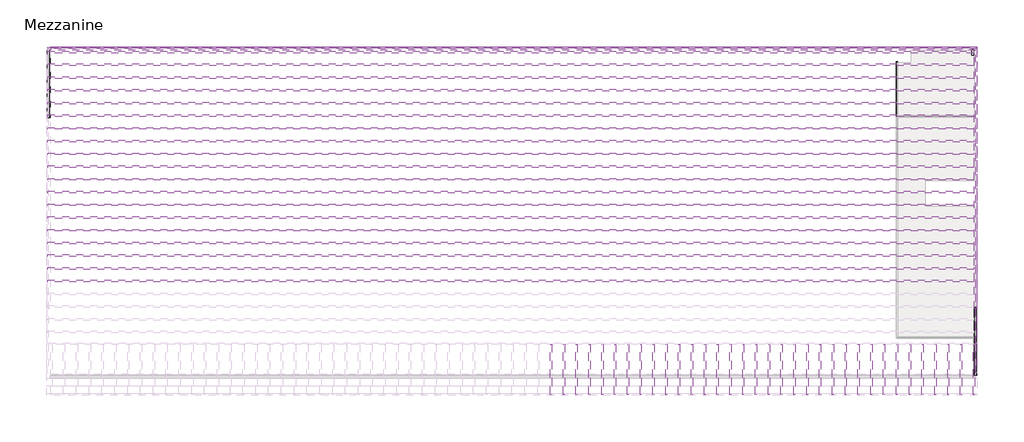
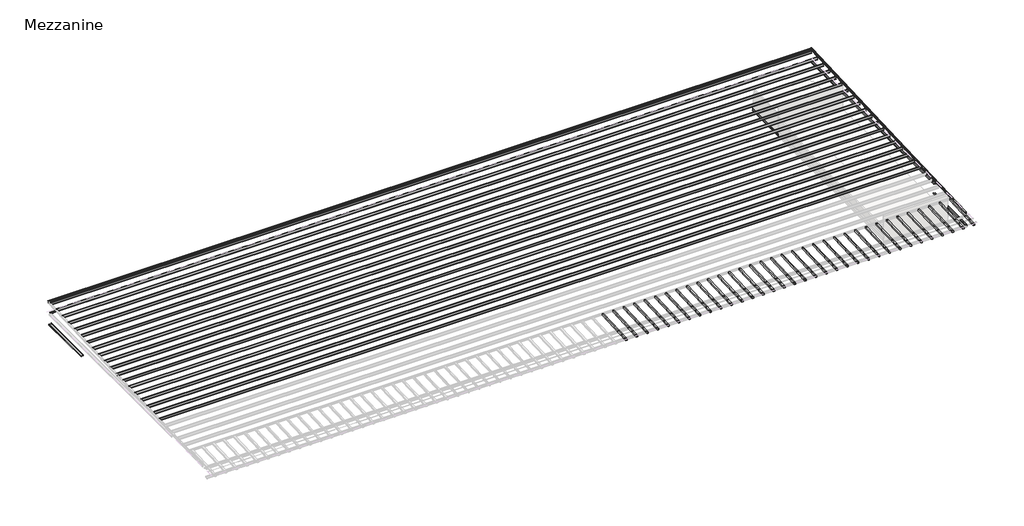
# One storey, part 2 of 2: 63 beams.
"""IFC4 building model written with IfcOpenShell, lengths in millimetres."""

import ifcopenshell
import ifcopenshell.guid

model = None  # the IFC model being written
_history = None  # IfcOwnerHistory: only IFC2X3 demands one
_inside = {}  # id of a spatial element -> (the spatial element, [elements in it])
_under = {}  # id of a project, library or spatial element -> (it, [spatial elements below it])
_declared = {}  # id of a project -> (the project, [libraries it declares])
_typed = {}  # id of a type object -> (the type object, [elements of that type])
_made_of = {}  # id of a material, layer set ... -> (it, [elements and type objects made of it])


def new_model(schema):
    """Start an empty IFC model of exactly this schema.

    Asked for "IFC4X3", IfcOpenShell would pick the latest addendum, in which some entities
    have other attributes; the version numbers below select the first issue.
    IFC2X3 requires an IfcOwnerHistory on every rooted entity: one is made here for all.
    """
    global model, _history
    if schema == "IFC4X3":
        model = ifcopenshell.file(schema_version=(4, 3, 0, 0))
    else:
        model = ifcopenshell.file(schema=schema)
    _inside.clear()
    _under.clear()
    _declared.clear()
    _typed.clear()
    _made_of.clear()
    _history = None
    if model.schema == "IFC2X3":
        org = make("IfcOrganization", Name="unknown")
        user = make(
            "IfcPersonAndOrganization",
            ThePerson=make("IfcPerson", FamilyName="unknown"),
            TheOrganization=org,
        )
        app = make(
            "IfcApplication",
            ApplicationDeveloper=org,
            Version="unknown",
            ApplicationFullName="unknown",
            ApplicationIdentifier="unknown",
        )
        _history = make(
            "IfcOwnerHistory",
            OwningUser=user,
            OwningApplication=app,
            ChangeAction="ADDED",
            CreationDate=0,
        )
    return model


def make(cls, **values):
    """One entity of the class cls with the attributes given. An attribute that is None is left unset."""
    return model.create_entity(
        cls, **{name: value for name, value in values.items() if value is not None}
    )


def rooted(cls, **values):
    """An entity with a GlobalId (a new one), such as an element, a storey or a relation."""
    return make(cls, GlobalId=ifcopenshell.guid.new(), OwnerHistory=_history, **values)


def si_unit(unit_type, name, prefix=None):
    """IfcSIUnit, for example si_unit("LENGTHUNIT", "METRE", prefix="MILLI")."""
    return make("IfcSIUnit", UnitType=unit_type, Prefix=prefix, Name=name)


def assignment(units):
    """IfcUnitAssignment: the units of a project."""
    return None if units is None else make("IfcUnitAssignment", Units=units)


def point(xyz):
    """IfcCartesianPoint."""
    return None if xyz is None else make("IfcCartesianPoint", Coordinates=xyz)


def direction(xyz):
    """IfcDirection."""
    return None if xyz is None else make("IfcDirection", DirectionRatios=xyz)


def frame(location, z_axis=None, x_axis=None):
    """IfcAxis2Placement3D, a coordinate frame: its origin and axes. An axis left out is left unset."""
    return make(
        "IfcAxis2Placement3D",
        Location=point(location),
        Axis=direction(z_axis),
        RefDirection=direction(x_axis),
    )


def frame_2d(location, x_axis=None):
    """IfcAxis2Placement2D, a coordinate frame in the plane: its origin and x axis."""
    return make(
        "IfcAxis2Placement2D", Location=point(location), RefDirection=direction(x_axis)
    )


def origin():
    """The frame at (0, 0, 0) with its axes left unset."""
    return frame((0.0, 0.0, 0.0))


def place(relative_to, where):
    """IfcLocalPlacement: puts the frame where relative to a parent placement (None: the world)."""
    return make(
        "IfcLocalPlacement", PlacementRelTo=relative_to, RelativePlacement=where
    )


def context(
    kind, dimensions, precision=None, world=None, true_north=None, identifier=None
):
    """IfcGeometricRepresentationContext, for example the 3D "Model" context."""
    return make(
        "IfcGeometricRepresentationContext",
        ContextIdentifier=identifier,
        ContextType=kind,
        CoordinateSpaceDimension=dimensions,
        Precision=precision,
        WorldCoordinateSystem=world,
        TrueNorth=true_north,
    )


def project(units=None, contexts=None):
    """IfcProject with its units and contexts."""
    return rooted(
        "IfcProject",
        Name="project",
        RepresentationContexts=contexts,
        UnitsInContext=assignment(units),
    )


def spatial(cls, under=None, at=None, **own):
    """A site, building, storey or space (cls), placed at a placement, below another one or the project."""
    s = rooted(cls, ObjectPlacement=at, **own)
    if under is not None:
        _under.setdefault(under.id(), (under, []))[1].append(s)
    return s


def polyline(points):
    """IfcPolyline through the points."""
    return make("IfcPolyline", Points=[point(p) for p in points])


def circle_curve(where, radius):
    """IfcCircle in the frame where."""
    return make("IfcCircle", Position=where, Radius=radius)


def trimmed(basis, trim1, trim2, sense, master):
    """IfcTrimmedCurve: the piece of a basis curve between two trims."""
    return make(
        "IfcTrimmedCurve",
        BasisCurve=basis,
        Trim1=trim1,
        Trim2=trim2,
        SenseAgreement=sense,
        MasterRepresentation=master,
    )


def segment(curve, same_sense, transition):
    """IfcCompositeCurveSegment."""
    return make(
        "IfcCompositeCurveSegment",
        Transition=transition,
        SameSense=same_sense,
        ParentCurve=curve,
    )


def composite_curve(segments, self_intersect=None):
    """IfcCompositeCurve: segments joined end to end."""
    return make("IfcCompositeCurve", Segments=segments, SelfIntersect=self_intersect)


def outline(outer, holes=None, kind="AREA"):
    """IfcArbitraryClosedProfileDef: a profile drawn as a closed curve; with holes, ...WithVoids."""
    if holes is None:
        return make("IfcArbitraryClosedProfileDef", ProfileType=kind, OuterCurve=outer)
    return make(
        "IfcArbitraryProfileDefWithVoids",
        ProfileType=kind,
        OuterCurve=outer,
        InnerCurves=holes,
    )


def extrude(swept, where, along, depth):
    """IfcExtrudedAreaSolid: the profile swept, set in the frame where, extruded along a direction by depth."""
    return make(
        "IfcExtrudedAreaSolid",
        SweptArea=swept,
        Position=where,
        ExtrudedDirection=direction(along),
        Depth=depth,
    )


def shape(context_of_items, identifier, shape_type, items):
    """IfcShapeRepresentation: the items that make up one representation, for example the "Body"."""
    return make(
        "IfcShapeRepresentation",
        ContextOfItems=context_of_items,
        RepresentationIdentifier=identifier,
        RepresentationType=shape_type,
        Items=items,
    )


def source(mapping_origin, context_of_items, identifier, shape_type, items):
    """IfcRepresentationMap: a shape defined once, which mapped items show again and again."""
    return make(
        "IfcRepresentationMap",
        MappingOrigin=mapping_origin,
        MappedRepresentation=shape(context_of_items, identifier, shape_type, items),
    )


def transform(
    local_origin,
    x_axis=None,
    y_axis=None,
    z_axis=None,
    scale=None,
    scale2=None,
    scale3=None,
    uniform=True,
):
    """IfcCartesianTransformationOperator3D, or its non-uniform kind. x_axis, y_axis, z_axis: its Axis1, 2, 3."""
    if uniform:
        return make(
            "IfcCartesianTransformationOperator3D",
            Axis1=direction(x_axis),
            Axis2=direction(y_axis),
            LocalOrigin=point(local_origin),
            Scale=scale,
            Axis3=direction(z_axis),
        )
    return make(
        "IfcCartesianTransformationOperator3DnonUniform",
        Axis1=direction(x_axis),
        Axis2=direction(y_axis),
        LocalOrigin=point(local_origin),
        Scale=scale,
        Axis3=direction(z_axis),
        Scale2=scale2,
        Scale3=scale3,
    )


def mapped(mapping_source, mapping_target):
    """IfcMappedItem: shows the shape of a source again, moved by a transform."""
    return make(
        "IfcMappedItem", MappingSource=mapping_source, MappingTarget=mapping_target
    )


def made_of(thing, what):
    """Note that an element or type object is made of a material, layer set ...; save() writes the relation."""
    if what is not None:
        _made_of.setdefault(what.id(), (what, []))[1].append(thing)
    return thing


def element(
    cls,
    number,
    at=None,
    inside=None,
    cuts=None,
    type_object=None,
    material=None,
    context=None,
    identifier="Body",
    shape_type=None,
    held_by="IfcProductDefinitionShape",
    body=None,
    shapes=None,
    **own,
):
    """One element of the class cls, such as IfcWall. Its Tag is "e" and its number.

    at: its placement. inside: the storey or other place that contains it. cuts: it is an
    opening in that element (IfcRelVoidsElement). A single representation is given by context,
    identifier, shape_type and body (its items); several are given by shapes. held_by: the class
    of the entity that holds the representations. save() writes the other relations.
    """
    e = rooted(cls, Tag="e%d" % number, ObjectPlacement=at, **own)
    if body is not None:
        shapes = [shape(context, identifier, shape_type, body)]
    if shapes is not None:
        e.Representation = make(held_by, Representations=shapes)
    if inside is not None:
        _inside.setdefault(inside.id(), (inside, []))[1].append(e)
    if cuts is not None:
        rooted(
            "IfcRelVoidsElement", RelatingBuildingElement=cuts, RelatedOpeningElement=e
        )
    if type_object is not None:
        _typed.setdefault(type_object.id(), (type_object, []))[1].append(e)
    return made_of(e, material)


def aggregate(whole, parts):
    """IfcRelAggregates: a whole, such as a stair, and the parts it consists of."""
    return rooted("IfcRelAggregates", RelatingObject=whole, RelatedObjects=parts)


def save(model, path):
    """Write the relations noted so far, then the file.

    IfcRelAggregates (storeys below a building ...), IfcRelContainedInSpatialStructure (elements
    in a storey), IfcRelDefinesByType, IfcRelAssociatesMaterial and IfcRelDeclares: one each for
    every whole, place, type object, material and project.
    """
    for whole, parts in _under.values():
        aggregate(whole, parts)
    for where, things in _inside.values():
        rooted(
            "IfcRelContainedInSpatialStructure",
            RelatedElements=things,
            RelatingStructure=where,
        )
    for kind, things in _typed.values():
        rooted("IfcRelDefinesByType", RelatedObjects=things, RelatingType=kind)
    for what, things in _made_of.values():
        rooted("IfcRelAssociatesMaterial", RelatedObjects=things, RelatingMaterial=what)
    for by, libraries in _declared.values():
        rooted("IfcRelDeclares", RelatingContext=by, RelatedDefinitions=libraries)
    model.write(path)


def dimension_lumber_5_5_x_7_5_glulam_5a1f9f63(model_context):
    return source(origin(), model_context, "Body", "SweptSolid", [
        extrude(outline(polyline([(2439.95575, 69.85), (2439.95575, -69.85), (-2389.02875, -69.85), (-2389.02875, 69.85), (2439.95575, 69.85)])), frame((0.0, 0.0, -95.25), z_axis=(0.0, 0.0, 1.0), x_axis=(1.0, 0.0, 0.0)), (0.0, 0.0, 1.0), 190.5),
    ])


def beam_8d9c0b98(model_context):
    return source(origin(), model_context, "Body", "SweptSolid", [
        extrude(outline(composite_curve([segment(polyline([(-87.5109375, 101.6), (-3.3734375, 101.6)]), True, "CONTINUOUS"), segment(trimmed(circle_curve(frame_2d((-3.3734375, 96.8375)), 4.7625), [point((-3.3734375, 101.6))], [point((1.3890625, 96.8375))], False, "CARTESIAN"), True, "CONTINUOUS"), segment(polyline([(1.3890625, 96.8375), (1.3890625, -96.8375)]), True, "CONTINUOUS"), segment(trimmed(circle_curve(frame_2d((-3.3734375, -96.8375)), 4.7625), [point((1.3890625, -96.8375))], [point((-3.3734375, -101.6))], False, "CARTESIAN"), True, "CONTINUOUS"), segment(polyline([(-3.3734375, -101.6), (-87.5109375, -101.6), (-99.7792647, -86.979177), (-97.6510975, -85.1934327), (-86.2154765, -98.821875), (-3.2694106, -98.821875)]), True, "CONTINUOUS"), segment(trimmed(circle_curve(frame_2d((-3.3748024, -96.8389339)), 1.9857399), [point((-3.2694106, -98.821875))], [point((-1.3890625, -96.8389339))], True, "CARTESIAN"), True, "CONTINUOUS"), segment(polyline([(-1.3890625, -96.8389339), (-1.3890625, 96.8381931)]), True, "CONTINUOUS"), segment(trimmed(circle_curve(frame_2d((-3.3741066, 96.8381931)), 1.9850441), [point((-1.3890625, 96.8381931))], [point((-3.3005807, 98.821875))], True, "CARTESIAN"), True, "CONTINUOUS"), segment(polyline([(-3.3005807, 98.821875), (-86.2154765, 98.821875), (-97.6278742, 85.221109), (-99.7560415, 87.0068534), (-87.5109375, 101.6)]), True, "CONTINUOUS")], self_intersect=False)), frame((-44450.0, 0.0, 0.0), z_axis=(1.0, 0.0, 0.0), x_axis=(0.0, 1.0, 0.0)), (0.0, 0.0, 1.0), 88900.0),
    ])


def beam_88a5fd93(model_context):
    return source(origin(), model_context, "Body", "SweptSolid", [
        extrude(outline(composite_curve([segment(polyline([(-87.5109375, 101.6), (-3.3734375, 101.6)]), True, "CONTINUOUS"), segment(trimmed(circle_curve(frame_2d((-3.3734375, 96.8375)), 4.7625), [point((-3.3734375, 101.6))], [point((1.3890625, 96.8375))], False, "CARTESIAN"), True, "CONTINUOUS"), segment(polyline([(1.3890625, 96.8375), (1.3890625, -96.8375)]), True, "CONTINUOUS"), segment(trimmed(circle_curve(frame_2d((-3.3734375, -96.8375)), 4.7625), [point((1.3890625, -96.8375))], [point((-3.3734375, -101.6))], False, "CARTESIAN"), True, "CONTINUOUS"), segment(polyline([(-3.3734375, -101.6), (-87.5109375, -101.6), (-99.7792647, -86.979177), (-97.6510975, -85.1934327), (-86.2154765, -98.821875), (-3.2694106, -98.821875)]), True, "CONTINUOUS"), segment(trimmed(circle_curve(frame_2d((-3.3748024, -96.8389339)), 1.9857399), [point((-3.2694106, -98.821875))], [point((-1.3890625, -96.8389339))], True, "CARTESIAN"), True, "CONTINUOUS"), segment(polyline([(-1.3890625, -96.8389339), (-1.3890625, 96.8381931)]), True, "CONTINUOUS"), segment(trimmed(circle_curve(frame_2d((-3.3741066, 96.8381931)), 1.9850441), [point((-1.3890625, 96.8381931))], [point((-3.3005807, 98.821875))], True, "CARTESIAN"), True, "CONTINUOUS"), segment(polyline([(-3.3005807, 98.821875), (-86.2154765, 98.821875), (-97.6278742, 85.221109), (-99.7560415, 87.0068534), (-87.5109375, 101.6)]), True, "CONTINUOUS")], self_intersect=False)), frame((-14148.6100916, 0.0, 0.0), z_axis=(1.0, 0.0, 0.0), x_axis=(0.0, 1.0, 0.0)), (0.0, 0.0, 1.0), 28297.2201833),
    ])


def beam_fb6f6511(model_context):
    return source(origin(), model_context, "Body", "SweptSolid", [
        extrude(outline(composite_curve([segment(polyline([(-87.5109375, 101.6), (-3.3734375, 101.6)]), True, "CONTINUOUS"), segment(trimmed(circle_curve(frame_2d((-3.3734375, 96.8375)), 4.7625), [point((-3.3734375, 101.6))], [point((1.3890625, 96.8375))], False, "CARTESIAN"), True, "CONTINUOUS"), segment(polyline([(1.3890625, 96.8375), (1.3890625, -96.8375)]), True, "CONTINUOUS"), segment(trimmed(circle_curve(frame_2d((-3.3734375, -96.8375)), 4.7625), [point((1.3890625, -96.8375))], [point((-3.3734375, -101.6))], False, "CARTESIAN"), True, "CONTINUOUS"), segment(polyline([(-3.3734375, -101.6), (-87.5109375, -101.6), (-99.7792647, -86.979177), (-97.6510975, -85.1934327), (-86.2154765, -98.821875), (-3.2694106, -98.821875)]), True, "CONTINUOUS"), segment(trimmed(circle_curve(frame_2d((-3.3748024, -96.8389339)), 1.9857399), [point((-3.2694106, -98.821875))], [point((-1.3890625, -96.8389339))], True, "CARTESIAN"), True, "CONTINUOUS"), segment(polyline([(-1.3890625, -96.8389339), (-1.3890625, 96.8381931)]), True, "CONTINUOUS"), segment(trimmed(circle_curve(frame_2d((-3.3741066, 96.8381931)), 1.9850441), [point((-1.3890625, 96.8381931))], [point((-3.3005807, 98.821875))], True, "CARTESIAN"), True, "CONTINUOUS"), segment(polyline([(-3.3005807, 98.821875), (-86.2154765, 98.821875), (-97.6278742, 85.221109), (-99.7560415, 87.0068534), (-87.5109375, 101.6)]), True, "CONTINUOUS")], self_intersect=False)), frame((-15570.2, 0.0, 0.0), z_axis=(1.0, 0.0, 0.0), x_axis=(0.0, 1.0, 0.0)), (0.0, 0.0, 1.0), 31140.4),
    ])


def beam_e6cd5542(model_context):
    return source(origin(), model_context, "Body", "SweptSolid", [
        extrude(outline(composite_curve([segment(polyline([(77.9859375, 127.0), (90.2310415, 112.4068534), (88.1028742, 110.621109), (76.6904765, 124.221875), (3.3005807, 124.221875)]), True, "CONTINUOUS"), segment(trimmed(circle_curve(frame_2d((3.3741066, 122.2381931)), 1.9850441), [point((3.3005807, 124.221875))], [point((1.3890625, 122.2381931))], True, "CARTESIAN"), True, "CONTINUOUS"), segment(polyline([(1.3890625, 122.2381931), (1.3890625, -127.0), (-84.3359375, -127.0), (-96.5810415, -112.4068534), (-94.4528742, -110.621109), (-83.0404765, -124.221875), (-3.2694106, -124.221875)]), True, "CONTINUOUS"), segment(trimmed(circle_curve(frame_2d((-3.3748024, -122.2389339)), 1.9857399), [point((-3.2694106, -124.221875))], [point((-1.3890625, -122.2389339))], True, "CARTESIAN"), True, "CONTINUOUS"), segment(polyline([(-1.3890625, -122.2389339), (-1.3890625, 122.2375)]), True, "CONTINUOUS"), segment(trimmed(circle_curve(frame_2d((3.3734375, 122.2375)), 4.7625), [point((-1.3890625, 122.2375))], [point((3.3734375, 127.0))], False, "CARTESIAN"), True, "CONTINUOUS"), segment(polyline([(3.3734375, 127.0), (77.9859375, 127.0)]), True, "CONTINUOUS")], self_intersect=False)), frame((-44224.90633, 0.0, 0.0), z_axis=(1.0, 0.0, 0.0), x_axis=(0.0, 1.0, 0.0)), (0.0, 0.0, 1.0), 88449.8126599),
    ])


def beam_3960b32e(model_context):
    return source(origin(), model_context, "Body", "SweptSolid", [
        extrude(outline(composite_curve([segment(polyline([(-77.9859375, 127.0), (-3.3734375, 127.0)]), True, "CONTINUOUS"), segment(trimmed(circle_curve(frame_2d((-3.3734375, 122.2375)), 4.7625), [point((-3.3734375, 127.0))], [point((1.3890625, 122.2375))], False, "CARTESIAN"), True, "CONTINUOUS"), segment(polyline([(1.3890625, 122.2375), (1.3890625, -122.2389339)]), True, "CONTINUOUS"), segment(trimmed(circle_curve(frame_2d((3.3748024, -122.2389339)), 1.9857399), [point((1.3890625, -122.2389339))], [point((3.2694106, -124.221875))], True, "CARTESIAN"), True, "CONTINUOUS"), segment(polyline([(3.2694106, -124.221875), (83.0404765, -124.221875), (94.4528742, -110.621109), (96.5810415, -112.4068534), (84.3359375, -127.0), (-1.3890625, -127.0), (-1.3890625, 122.2381931)]), True, "CONTINUOUS"), segment(trimmed(circle_curve(frame_2d((-3.3741066, 122.2381931)), 1.9850441), [point((-1.3890625, 122.2381931))], [point((-3.3005807, 124.221875))], True, "CARTESIAN"), True, "CONTINUOUS"), segment(polyline([(-3.3005807, 124.221875), (-76.6904765, 124.221875), (-88.1028742, 110.621109), (-90.2310415, 112.4068534), (-77.9859375, 127.0)]), True, "CONTINUOUS")], self_intersect=False)), frame((-3235.325, 0.0, 0.0), z_axis=(1.0, 0.0, 0.0), x_axis=(0.0, 1.0, 0.0)), (0.0, 0.0, 1.0), 6470.65),
    ])


def beam_08c7dc4f(model_context):
    return source(origin(), model_context, "Body", "SweptSolid", [
        extrude(outline(composite_curve([segment(polyline([(-77.9859375, 127.0), (-3.3734375, 127.0)]), True, "CONTINUOUS"), segment(trimmed(circle_curve(frame_2d((-3.3734375, 122.2375)), 4.7625), [point((-3.3734375, 127.0))], [point((1.3890625, 122.2375))], False, "CARTESIAN"), True, "CONTINUOUS"), segment(polyline([(1.3890625, 122.2375), (1.3890625, -122.2389339)]), True, "CONTINUOUS"), segment(trimmed(circle_curve(frame_2d((3.3748024, -122.2389339)), 1.9857399), [point((1.3890625, -122.2389339))], [point((3.2694106, -124.221875))], True, "CARTESIAN"), True, "CONTINUOUS"), segment(polyline([(3.2694106, -124.221875), (83.0404765, -124.221875), (94.4528742, -110.621109), (96.5810415, -112.4068534), (84.3359375, -127.0), (-1.3890625, -127.0), (-1.3890625, 122.2381931)]), True, "CONTINUOUS"), segment(trimmed(circle_curve(frame_2d((-3.3741066, 122.2381931)), 1.9850441), [point((-1.3890625, 122.2381931))], [point((-3.3005807, 124.221875))], True, "CARTESIAN"), True, "CONTINUOUS"), segment(polyline([(-3.3005807, 124.221875), (-76.6904765, 124.221875), (-88.1028742, 110.621109), (-90.2310415, 112.4068534), (-77.9859375, 127.0)]), True, "CONTINUOUS")], self_intersect=False)), frame((-12376.1500241, 0.0, 0.0), z_axis=(1.0, 0.0, 0.0), x_axis=(0.0, 1.0, 0.0)), (0.0, 0.0, 1.0), 24752.3000483),
    ])


def beam_44ace1b0(model_context):
    return source(origin(), model_context, "Body", "SweptSolid", [
        extrude(outline(composite_curve([segment(polyline([(77.9859375, 127.0), (90.2310415, 112.4068534), (88.1028742, 110.621109), (76.6904765, 124.221875), (3.3005807, 124.221875)]), True, "CONTINUOUS"), segment(trimmed(circle_curve(frame_2d((3.3741066, 122.2381931)), 1.9850441), [point((3.3005807, 124.221875))], [point((1.3890625, 122.2381931))], True, "CARTESIAN"), True, "CONTINUOUS"), segment(polyline([(1.3890625, 122.2381931), (1.3890625, -127.0), (-84.3359375, -127.0), (-96.5810415, -112.4068534), (-94.4528742, -110.621109), (-83.0404765, -124.221875), (-3.2694106, -124.221875)]), True, "CONTINUOUS"), segment(trimmed(circle_curve(frame_2d((-3.3748024, -122.2389339)), 1.9857399), [point((-3.2694106, -124.221875))], [point((-1.3890625, -122.2389339))], True, "CARTESIAN"), True, "CONTINUOUS"), segment(polyline([(-1.3890625, -122.2389339), (-1.3890625, 122.2375)]), True, "CONTINUOUS"), segment(trimmed(circle_curve(frame_2d((3.3734375, 122.2375)), 4.7625), [point((-1.3890625, 122.2375))], [point((3.3734375, 127.0))], False, "CARTESIAN"), True, "CONTINUOUS"), segment(polyline([(3.3734375, 127.0), (77.9859375, 127.0)]), True, "CONTINUOUS")], self_intersect=False)), frame((-3314.7, 0.0, 0.0), z_axis=(1.0, 0.0, 0.0), x_axis=(0.0, 1.0, 0.0)), (0.0, 0.0, 1.0), 6470.65),
    ])


def beam_bf61a610(model_context):
    return source(origin(), model_context, "Body", "SweptSolid", [
        extrude(outline(composite_curve([segment(polyline([(77.9859375, 127.0), (90.2310415, 112.4068534), (88.1028742, 110.621109), (76.6904765, 124.221875), (3.3005807, 124.221875)]), True, "CONTINUOUS"), segment(trimmed(circle_curve(frame_2d((3.3741066, 122.2381931)), 1.9850441), [point((3.3005807, 124.221875))], [point((1.3890625, 122.2381931))], True, "CARTESIAN"), True, "CONTINUOUS"), segment(polyline([(1.3890625, 122.2381931), (1.3890625, -127.0), (-84.3359375, -127.0), (-96.5810415, -112.4068534), (-94.4528742, -110.621109), (-83.0404765, -124.221875), (-3.2694106, -124.221875)]), True, "CONTINUOUS"), segment(trimmed(circle_curve(frame_2d((-3.3748024, -122.2389339)), 1.9857399), [point((-3.2694106, -124.221875))], [point((-1.3890625, -122.2389339))], True, "CARTESIAN"), True, "CONTINUOUS"), segment(polyline([(-1.3890625, -122.2389339), (-1.3890625, 122.2375)]), True, "CONTINUOUS"), segment(trimmed(circle_curve(frame_2d((3.3734375, 122.2375)), 4.7625), [point((-1.3890625, 122.2375))], [point((3.3734375, 127.0))], False, "CARTESIAN"), True, "CONTINUOUS"), segment(polyline([(3.3734375, 127.0), (77.9859375, 127.0)]), True, "CONTINUOUS")], self_intersect=False)), frame((-44283.1884767, 0.0, 0.0), z_axis=(1.0, 0.0, 0.0), x_axis=(0.0, 1.0, 0.0)), (0.0, 0.0, 1.0), 88566.3769533),
    ])


def l_angle_l2x2x3_16_9da130ac(model_context):
    return source(origin(), model_context, "Body", "SweptSolid", [
        extrude(outline(composite_curve([segment(polyline([(-14.2494, 14.2494), (36.5506, 14.2494)]), True, "CONTINUOUS"), segment(trimmed(circle_curve(frame_2d((31.7881, 14.2494)), 4.7625), [point((36.5506, 14.2494))], [point((31.7881, 9.4869))], False, "CARTESIAN"), True, "CONTINUOUS"), segment(polyline([(31.7881, 9.4869), (-4.7244, 9.4869)]), True, "CONTINUOUS"), segment(trimmed(circle_curve(frame_2d((-4.7244, 4.7244)), 4.7625), [point((-4.7244, 9.4869))], [point((-9.4869, 4.7244))], True, "CARTESIAN"), True, "CONTINUOUS"), segment(polyline([(-9.4869, 4.7244), (-9.4869, -31.7881)]), True, "CONTINUOUS"), segment(trimmed(circle_curve(frame_2d((-14.2494, -31.7881)), 4.7625), [point((-9.4869, -31.7881))], [point((-14.2494, -36.5506))], False, "CARTESIAN"), True, "CONTINUOUS"), segment(polyline([(-14.2494, -36.5506), (-14.2494, 14.2494)]), True, "CONTINUOUS")], self_intersect=False)), frame((-44322.7519531, 0.0, 0.0), z_axis=(1.0, 0.0, 0.0), x_axis=(0.0, 1.0, 0.0)), (0.0, 0.0, 1.0), 88645.5039063),
    ])


def w_wide_flange_w12x26_6f15523d(model_context):
    return source(origin(), model_context, "Body", "SweptSolid", [
        extrude(outline(composite_curve([segment(polyline([(82.4011719, -145.5539063), (82.4011719, -155.178125), (-82.4011719, -155.178125), (-82.4011719, -145.5539063), (-20.2902344, -145.5539063)]), True, "CONTINUOUS"), segment(trimmed(circle_curve(frame_2d((-20.2902344, -128.190625)), 17.3632812), [point((-20.2902344, -145.5539063))], [point((-2.9269531, -128.190625))], True, "CARTESIAN"), True, "CONTINUOUS"), segment(polyline([(-2.9269531, -128.190625), (-2.9269531, 128.190625)]), True, "CONTINUOUS"), segment(trimmed(circle_curve(frame_2d((-20.2902344, 128.190625)), 17.3632812), [point((-2.9269531, 128.190625))], [point((-20.2902344, 145.5539062))], True, "CARTESIAN"), True, "CONTINUOUS"), segment(polyline([(-20.2902344, 145.5539062), (-82.4011719, 145.5539062), (-82.4011719, 155.178125), (82.4011719, 155.178125), (82.4011719, 145.5539062), (20.2902344, 145.5539062)]), True, "CONTINUOUS"), segment(trimmed(circle_curve(frame_2d((20.2902344, 128.190625)), 17.3632812), [point((20.2902344, 145.5539062))], [point((2.9269531, 128.190625))], True, "CARTESIAN"), True, "CONTINUOUS"), segment(polyline([(2.9269531, 128.190625), (2.9269531, -128.190625)]), True, "CONTINUOUS"), segment(trimmed(circle_curve(frame_2d((20.2902344, -128.190625)), 17.3632812), [point((2.9269531, -128.190625))], [point((20.2902344, -145.5539063))], True, "CARTESIAN"), True, "CONTINUOUS"), segment(polyline([(20.2902344, -145.5539063), (82.4011719, -145.5539063)]), True, "CONTINUOUS")], self_intersect=False)), frame((-2633.8467178, 0.0, 0.0), z_axis=(1.0, 0.0, 0.0), x_axis=(0.0, 1.0, 0.0)), (0.0, 0.0, 1.0), 5267.6934356),
    ])


def w_wide_flange_w12x26_3769b023(model_context):
    return source(origin(), model_context, "Body", "SweptSolid", [
        extrude(outline(composite_curve([segment(polyline([(82.4011719, -145.5539063), (82.4011719, -155.178125), (-82.4011719, -155.178125), (-82.4011719, -145.5539063), (-20.2902344, -145.5539063)]), True, "CONTINUOUS"), segment(trimmed(circle_curve(frame_2d((-20.2902344, -128.190625)), 17.3632812), [point((-20.2902344, -145.5539063))], [point((-2.9269531, -128.190625))], True, "CARTESIAN"), True, "CONTINUOUS"), segment(polyline([(-2.9269531, -128.190625), (-2.9269531, 128.190625)]), True, "CONTINUOUS"), segment(trimmed(circle_curve(frame_2d((-20.2902344, 128.190625)), 17.3632812), [point((-2.9269531, 128.190625))], [point((-20.2902344, 145.5539062))], True, "CARTESIAN"), True, "CONTINUOUS"), segment(polyline([(-20.2902344, 145.5539062), (-82.4011719, 145.5539062), (-82.4011719, 155.178125), (82.4011719, 155.178125), (82.4011719, 145.5539062), (20.2902344, 145.5539062)]), True, "CONTINUOUS"), segment(trimmed(circle_curve(frame_2d((20.2902344, 128.190625)), 17.3632812), [point((20.2902344, 145.5539062))], [point((2.9269531, 128.190625))], True, "CARTESIAN"), True, "CONTINUOUS"), segment(polyline([(2.9269531, 128.190625), (2.9269531, -128.190625)]), True, "CONTINUOUS"), segment(trimmed(circle_curve(frame_2d((20.2902344, -128.190625)), 17.3632812), [point((2.9269531, -128.190625))], [point((20.2902344, -145.5539063))], True, "CARTESIAN"), True, "CONTINUOUS"), segment(polyline([(20.2902344, -145.5539063), (82.4011719, -145.5539063)]), True, "CONTINUOUS")], self_intersect=False)), frame((-3333.7106844, 0.0, 0.0), z_axis=(1.0, 0.0, 0.0), x_axis=(0.0, 1.0, 0.0)), (0.0, 0.0, 1.0), 6397.5856844),
    ])


model = new_model("IFC4")

# Units and contexts
model_context = context("Model", 3, world=origin())
ifc_project = project(units=[si_unit("LENGTHUNIT", "METRE", prefix="MILLI")], contexts=[model_context])

# Site, building, storey
site = spatial("IfcSite", under=ifc_project)
building = spatial("IfcBuilding", under=site)
storey = spatial("IfcBuildingStorey", under=building, Name="Mezzanine", Elevation=6553.2)

# Beams
placement = place(None, origin())
dimension_lumber_5_5_x_7_5_glulam_shape = dimension_lumber_5_5_x_7_5_glulam_5a1f9f63(model_context)
element("IfcBeam", 1, ObjectType="Dimension Lumber : 5.5 x 7.5 Glulam", at=placement, inside=storey, context=model_context, shape_type="MappedRepresentation", body=[
    mapped(dimension_lumber_5_5_x_7_5_glulam_shape, transform((667267.9117243, -567351.2774558, 8705.0370798), x_axis=(0.0, -0.999133073092352, -0.04163054471217889), y_axis=(1.0, 0.0, 0.0), z_axis=(0.0, -0.0416305447121789, 0.9991330730923521))),
])
element("IfcBeam", 2, ObjectType="Dimension Lumber : 5.5 x 7.5 Glulam", at=placement, inside=storey, context=model_context, shape_type="MappedRepresentation", body=[
    mapped(dimension_lumber_5_5_x_7_5_glulam_shape, transform((666042.3617243, -567351.2774558, 8705.0370798), x_axis=(0.0, -0.999133073092352, -0.04163054471217911), y_axis=(1.0, 0.0, 0.0), z_axis=(0.0, -0.04163054471217912, 0.9991330730923521))),
])
element("IfcBeam", 3, ObjectType="Dimension Lumber : 5.5 x 7.5 Glulam", at=placement, inside=storey, context=model_context, shape_type="MappedRepresentation", body=[
    mapped(dimension_lumber_5_5_x_7_5_glulam_shape, transform((664816.8117243, -567351.2774558, 8705.0370798), x_axis=(0.0, -0.999133073092352, -0.04163054471217889), y_axis=(1.0, 0.0, 0.0), z_axis=(0.0, -0.0416305447121789, 0.9991330730923521))),
])
element("IfcBeam", 4, ObjectType="Dimension Lumber : 5.5 x 7.5 Glulam", at=placement, inside=storey, context=model_context, shape_type="MappedRepresentation", body=[
    mapped(dimension_lumber_5_5_x_7_5_glulam_shape, transform((663591.2617243, -567351.2774558, 8705.0370798), x_axis=(0.0, -0.999133073092352, -0.04163054471217889), y_axis=(1.0, 0.0, 0.0), z_axis=(0.0, -0.0416305447121789, 0.9991330730923521))),
])
element("IfcBeam", 5, ObjectType="Dimension Lumber : 5.5 x 7.5 Glulam", at=placement, inside=storey, context=model_context, shape_type="MappedRepresentation", body=[
    mapped(dimension_lumber_5_5_x_7_5_glulam_shape, transform((662365.7117243, -567351.2774558, 8705.0370798), x_axis=(0.0, -0.999133073092352, -0.04163054471217911), y_axis=(1.0, 0.0, 0.0), z_axis=(0.0, -0.04163054471217912, 0.9991330730923521))),
])
element("IfcBeam", 6, ObjectType="Dimension Lumber : 5.5 x 7.5 Glulam", at=placement, inside=storey, context=model_context, shape_type="MappedRepresentation", body=[
    mapped(dimension_lumber_5_5_x_7_5_glulam_shape, transform((661140.1617243, -567351.2774558, 8705.0370798), x_axis=(0.0, -0.999133073092352, -0.04163054471217889), y_axis=(1.0, 0.0, 0.0), z_axis=(0.0, -0.041630544712178974, 0.9991330730923521))),
])
element("IfcBeam", 7, ObjectType="Dimension Lumber : 5.5 x 7.5 Glulam", at=placement, inside=storey, context=model_context, shape_type="MappedRepresentation", body=[
    mapped(dimension_lumber_5_5_x_7_5_glulam_shape, transform((659914.6117243, -567351.2774558, 8705.0370798), x_axis=(0.0, -0.999133073092352, -0.04163054471217889), y_axis=(1.0, 0.0, 0.0), z_axis=(0.0, -0.0416305447121789, 0.9991330730923521))),
])
element("IfcBeam", 8, ObjectType="Dimension Lumber : 5.5 x 7.5 Glulam", at=placement, inside=storey, context=model_context, shape_type="MappedRepresentation", body=[
    mapped(dimension_lumber_5_5_x_7_5_glulam_shape, transform((658689.0617243, -567351.2774558, 8705.0370798), x_axis=(0.0, -0.999133073092352, -0.04163054471217911), y_axis=(1.0, 0.0, 0.0), z_axis=(0.0, -0.04163054471217912, 0.9991330730923521))),
])
element("IfcBeam", 9, ObjectType="Dimension Lumber : 5.5 x 7.5 Glulam", at=placement, inside=storey, context=model_context, shape_type="MappedRepresentation", body=[
    mapped(dimension_lumber_5_5_x_7_5_glulam_shape, transform((657463.5117243, -567351.2774558, 8705.0370798), x_axis=(0.0, -0.999133073092352, -0.04163054471217889), y_axis=(1.0, 0.0, 0.0), z_axis=(0.0, -0.041630544712178974, 0.9991330730923521))),
])
element("IfcBeam", 10, ObjectType="Dimension Lumber : 5.5 x 7.5 Glulam", at=placement, inside=storey, context=model_context, shape_type="MappedRepresentation", body=[
    mapped(dimension_lumber_5_5_x_7_5_glulam_shape, transform((656237.9617243, -567351.2774558, 8705.0370798), x_axis=(0.0, -0.999133073092352, -0.04163054471217889), y_axis=(1.0, 0.0, 0.0), z_axis=(0.0, -0.0416305447121789, 0.9991330730923521))),
])
element("IfcBeam", 11, ObjectType="Dimension Lumber : 5.5 x 7.5 Glulam", at=placement, inside=storey, context=model_context, shape_type="MappedRepresentation", body=[
    mapped(dimension_lumber_5_5_x_7_5_glulam_shape, transform((655012.4117243, -567351.2774558, 8705.0370798), x_axis=(0.0, -0.999133073092352, -0.04163054471217911), y_axis=(0.9999999999999999, 0.0, 0.0), z_axis=(0.0, -0.04163054471217918, 0.999133073092352))),
])
element("IfcBeam", 12, ObjectType="Dimension Lumber : 5.5 x 7.5 Glulam", at=placement, inside=storey, context=model_context, shape_type="MappedRepresentation", body=[
    mapped(dimension_lumber_5_5_x_7_5_glulam_shape, transform((653786.8617243, -567351.2774558, 8705.0370798), x_axis=(0.0, -0.999133073092352, -0.04163054471217889), y_axis=(1.0, 0.0, 0.0), z_axis=(0.0, -0.041630544712178974, 0.9991330730923521))),
])
element("IfcBeam", 13, ObjectType="Dimension Lumber : 5.5 x 7.5 Glulam", at=placement, inside=storey, context=model_context, shape_type="MappedRepresentation", body=[
    mapped(dimension_lumber_5_5_x_7_5_glulam_shape, transform((652561.3117243, -567351.2774558, 8705.0370798), x_axis=(0.0, -0.999133073092352, -0.04163054471217889), y_axis=(1.0, 0.0, 0.0), z_axis=(0.0, -0.0416305447121789, 0.9991330730923521))),
])
element("IfcBeam", 14, ObjectType="Dimension Lumber : 5.5 x 7.5 Glulam", at=placement, inside=storey, context=model_context, shape_type="MappedRepresentation", body=[
    mapped(dimension_lumber_5_5_x_7_5_glulam_shape, transform((651335.7617243, -567351.2774558, 8705.0370798), x_axis=(0.0, -0.999133073092352, -0.04163054471217911), y_axis=(0.9999999999999999, 0.0, 0.0), z_axis=(0.0, -0.04163054471217918, 0.999133073092352))),
])
element("IfcBeam", 15, ObjectType="Dimension Lumber : 5.5 x 7.5 Glulam", at=placement, inside=storey, context=model_context, shape_type="MappedRepresentation", body=[
    mapped(dimension_lumber_5_5_x_7_5_glulam_shape, transform((650110.2117243, -567351.2774558, 8705.0370798), x_axis=(0.0, -0.999133073092352, -0.04163054471217889), y_axis=(1.0, 0.0, 0.0), z_axis=(0.0, -0.041630544712178974, 0.9991330730923521))),
])
element("IfcBeam", 16, ObjectType="Dimension Lumber : 5.5 x 7.5 Glulam", at=placement, inside=storey, context=model_context, shape_type="MappedRepresentation", body=[
    mapped(dimension_lumber_5_5_x_7_5_glulam_shape, transform((648884.6617243, -567351.2774558, 8705.0370798), x_axis=(0.0, -0.999133073092352, -0.04163054471217889), y_axis=(1.0, 0.0, 0.0), z_axis=(0.0, -0.0416305447121789, 0.9991330730923521))),
])
element("IfcBeam", 17, ObjectType="Dimension Lumber : 5.5 x 7.5 Glulam", at=placement, inside=storey, context=model_context, shape_type="MappedRepresentation", body=[
    mapped(dimension_lumber_5_5_x_7_5_glulam_shape, transform((647659.1117243, -567351.2774558, 8705.0370798), x_axis=(0.0, -0.999133073092352, -0.04163054471217911), y_axis=(0.9999999999999999, 0.0, 0.0), z_axis=(0.0, -0.04163054471217918, 0.999133073092352))),
])
element("IfcBeam", 18, ObjectType="Dimension Lumber : 5.5 x 7.5 Glulam", at=placement, inside=storey, context=model_context, shape_type="MappedRepresentation", body=[
    mapped(dimension_lumber_5_5_x_7_5_glulam_shape, transform((646433.5617243, -567351.2774558, 8705.0370798), x_axis=(0.0, -0.999133073092352, -0.04163054471217889), y_axis=(1.0, 0.0, 0.0), z_axis=(0.0, -0.041630544712178974, 0.9991330730923521))),
])
element("IfcBeam", 19, ObjectType="Dimension Lumber : 5.5 x 7.5 Glulam", at=placement, inside=storey, context=model_context, shape_type="MappedRepresentation", body=[
    mapped(dimension_lumber_5_5_x_7_5_glulam_shape, transform((645208.0117243, -567351.2774558, 8705.0370798), x_axis=(0.0, -0.999133073092352, -0.04163054471217889), y_axis=(1.0, 0.0, 0.0), z_axis=(0.0, -0.04163054471217882, 0.9991330730923521))),
])
element("IfcBeam", 20, ObjectType="Dimension Lumber : 5.5 x 7.5 Glulam", at=placement, inside=storey, context=model_context, shape_type="MappedRepresentation", body=[
    mapped(dimension_lumber_5_5_x_7_5_glulam_shape, transform((643982.4617243, -567351.2774558, 8705.0370798), x_axis=(0.0, -0.999133073092352, -0.04163054471217889), y_axis=(1.0, 0.0, 0.0), z_axis=(0.0, -0.041630544712178974, 0.9991330730923521))),
])
element("IfcBeam", 21, ObjectType="Dimension Lumber : 5.5 x 7.5 Glulam", at=placement, inside=storey, context=model_context, shape_type="MappedRepresentation", body=[
    mapped(dimension_lumber_5_5_x_7_5_glulam_shape, transform((642756.9117243, -567351.2774558, 8705.0370798), x_axis=(0.0, -0.999133073092352, -0.04163054471217889), y_axis=(1.0, 0.0, 0.0), z_axis=(0.0, -0.041630544712178974, 0.9991330730923521))),
])
element("IfcBeam", 22, ObjectType="Dimension Lumber : 5.5 x 7.5 Glulam", at=placement, inside=storey, context=model_context, shape_type="MappedRepresentation", body=[
    mapped(dimension_lumber_5_5_x_7_5_glulam_shape, transform((641531.3617243, -567351.2774558, 8705.0370798), x_axis=(0.0, -0.999133073092352, -0.04163054471217911), y_axis=(1.0, 0.0, 0.0), z_axis=(0.0, -0.04163054471217904, 0.9991330730923521))),
])
element("IfcBeam", 23, ObjectType="Dimension Lumber : 5.5 x 7.5 Glulam", at=placement, inside=storey, context=model_context, shape_type="MappedRepresentation", body=[
    mapped(dimension_lumber_5_5_x_7_5_glulam_shape, transform((640305.8117243, -567351.2774558, 8705.0370798), x_axis=(0.0, -0.999133073092352, -0.04163054471217889), y_axis=(1.0, 0.0, 0.0), z_axis=(0.0, -0.041630544712178974, 0.9991330730923521))),
])
element("IfcBeam", 24, ObjectType="Dimension Lumber : 5.5 x 7.5 Glulam", at=placement, inside=storey, context=model_context, shape_type="MappedRepresentation", body=[
    mapped(dimension_lumber_5_5_x_7_5_glulam_shape, transform((639080.2617243, -567351.2774558, 8705.0370798), x_axis=(0.0, -0.999133073092352, -0.04163054471217889), y_axis=(1.0, 0.0, 0.0), z_axis=(0.0, -0.04163054471217882, 0.9991330730923521))),
])
element("IfcBeam", 25, ObjectType="Dimension Lumber : 5.5 x 7.5 Glulam", at=placement, inside=storey, context=model_context, shape_type="MappedRepresentation", body=[
    mapped(dimension_lumber_5_5_x_7_5_glulam_shape, transform((637854.7117243, -567351.2774558, 8705.0370798), x_axis=(0.0, -0.999133073092352, -0.04163054471217911), y_axis=(1.0, 0.0, 0.0), z_axis=(0.0, -0.04163054471217904, 0.9991330730923521))),
])
element("IfcBeam", 26, ObjectType="Dimension Lumber : 5.5 x 7.5 Glulam", at=placement, inside=storey, context=model_context, shape_type="MappedRepresentation", body=[
    mapped(dimension_lumber_5_5_x_7_5_glulam_shape, transform((636629.1617243, -567351.2774558, 8705.0370798), x_axis=(0.0, -0.999133073092352, -0.04163054471217889), y_axis=(1.0, 0.0, 0.0), z_axis=(0.0, -0.041630544712178974, 0.9991330730923521))),
])
element("IfcBeam", 27, ObjectType="Dimension Lumber : 5.5 x 7.5 Glulam", at=placement, inside=storey, context=model_context, shape_type="MappedRepresentation", body=[
    mapped(dimension_lumber_5_5_x_7_5_glulam_shape, transform((635403.6117243, -567351.2774558, 8705.0370798), x_axis=(0.0, -0.999133073092352, -0.04163054471217889), y_axis=(1.0, 0.0, 0.0), z_axis=(0.0, -0.04163054471217882, 0.9991330730923521))),
])
element("IfcBeam", 28, ObjectType="Dimension Lumber : 5.5 x 7.5 Glulam", at=placement, inside=storey, context=model_context, shape_type="MappedRepresentation", body=[
    mapped(dimension_lumber_5_5_x_7_5_glulam_shape, transform((634178.0617243, -567351.2774558, 8705.0370798), x_axis=(0.0, -0.999133073092352, -0.04163054471217911), y_axis=(1.0, 0.0, 0.0), z_axis=(0.0, -0.04163054471217904, 0.9991330730923521))),
])
element("IfcBeam", 29, ObjectType="Dimension Lumber : 5.5 x 7.5 Glulam", at=placement, inside=storey, context=model_context, shape_type="MappedRepresentation", body=[
    mapped(dimension_lumber_5_5_x_7_5_glulam_shape, transform((632952.5117243, -567351.2774558, 8705.0370798), x_axis=(0.0, -0.999133073092352, -0.04163054471217889), y_axis=(1.0, 0.0, 0.0), z_axis=(0.0, -0.041630544712178974, 0.9991330730923521))),
])
element("IfcBeam", 30, ObjectType="Dimension Lumber : 5.5 x 7.5 Glulam", at=placement, inside=storey, context=model_context, shape_type="MappedRepresentation", body=[
    mapped(dimension_lumber_5_5_x_7_5_glulam_shape, transform((631726.9617243, -567351.2774558, 8705.0370798), x_axis=(0.0, -0.999133073092352, -0.04163054471217889), y_axis=(1.0, 0.0, 0.0), z_axis=(0.0, -0.04163054471217882, 0.9991330730923521))),
])
element("IfcBeam", 31, ObjectType="Dimension Lumber : 5.5 x 7.5 Glulam", at=placement, inside=storey, context=model_context, shape_type="MappedRepresentation", body=[
    mapped(dimension_lumber_5_5_x_7_5_glulam_shape, transform((630501.4117243, -567351.2774558, 8705.0370798), x_axis=(0.0, -0.999133073092352, -0.04163054471217911), y_axis=(1.0, 0.0, 0.0), z_axis=(0.0, -0.04163054471217904, 0.9991330730923521))),
])
element("IfcBeam", 32, ObjectType="Dimension Lumber : 5.5 x 7.5 Glulam", at=placement, inside=storey, context=model_context, shape_type="MappedRepresentation", body=[
    mapped(dimension_lumber_5_5_x_7_5_glulam_shape, transform((629275.8617243, -567351.2774558, 8705.0370798), x_axis=(0.0, -0.999133073092352, -0.04163054471217889), y_axis=(1.0, 0.0, 0.0), z_axis=(0.0, -0.04163054471217882, 0.9991330730923521))),
])
element("IfcBeam", 33, ObjectType="Dimension Lumber : 5.5 x 7.5 Glulam", at=placement, inside=storey, context=model_context, shape_type="MappedRepresentation", body=[
    mapped(dimension_lumber_5_5_x_7_5_glulam_shape, transform((628050.3117243, -567351.2774558, 8705.0370798), x_axis=(0.0, -0.999133073092352, -0.04163054471217889), y_axis=(1.0, 0.0, 0.0), z_axis=(0.0, -0.04163054471217882, 0.9991330730923521))),
])
element("IfcBeam", 34, ObjectType="Dimension Lumber : 5.5 x 7.5 Glulam", at=placement, inside=storey, context=model_context, shape_type="MappedRepresentation", body=[
    mapped(dimension_lumber_5_5_x_7_5_glulam_shape, transform((626824.7617243, -567351.2774558, 8705.0370798), x_axis=(0.0, -0.999133073092352, -0.04163054471217911), y_axis=(1.0, 0.0, 0.0), z_axis=(0.0, -0.04163054471217904, 0.9991330730923521))),
])
beam_shape = beam_8d9c0b98(model_context)
element("IfcBeam", 35, ObjectType="Girt_C : 8\"D", at=placement, inside=storey, context=model_context, shape_type="MappedRepresentation", body=[
    mapped(beam_shape, transform((623097.3117239, -536558.6804466, 9994.5634988), x_axis=(1.0, 0.0, 0.0), y_axis=(0.0, 1.0, 0.0), z_axis=(0.0, 0.0, 1.0))),
])
beam_2_shape = beam_88a5fd93(model_context)
element("IfcBeam", 36, ObjectType="Girt_C : 8\"D", at=placement, inside=storey, context=model_context, shape_type="MappedRepresentation", body=[
    mapped(beam_2_shape, transform((667547.3117239, -550703.8827187, 9405.034037), x_axis=(0.0, -0.9991330730923521, -0.04163054471217908), y_axis=(1.0000000000000002, 0.0, 0.0), z_axis=(0.0, -0.04163054471217907, 0.9991330730923521))),
])
beam_3_shape = beam_fb6f6511(model_context)
element("IfcBeam", 37, ObjectType="Girt_C : 8\"D", at=placement, inside=storey, context=model_context, shape_type="MappedRepresentation", body=[
    mapped(beam_3_shape, transform((667545.9226614, -552151.2369713, 9344.7276098), x_axis=(0.0, -0.9991330730923521, -0.04163054471217908), y_axis=(1.0000000000000002, 0.0, 0.0), z_axis=(0.0, -0.04163054471217909, 0.9991330730923521))),
])
beam_4_shape = beam_e6cd5542(model_context)
element("IfcBeam", 38, ObjectType="Girt_Z : 10\"D", at=placement, inside=storey, context=model_context, shape_type="MappedRepresentation", body=[
    mapped(beam_4_shape, transform((623227.1553939, -536684.2899502, 8578.6515625), x_axis=(1.0000000000000002, 0.0, 0.0), y_axis=(0.0, 0.0, -1.0000000000000002), z_axis=(0.0, 1.0000000000000002, 0.0))),
])
beam_5_shape = beam_3960b32e(model_context)
element("IfcBeam", 39, ObjectType="Girt_Z : 10\"D", at=placement, inside=storey, context=model_context, shape_type="MappedRepresentation", body=[
    mapped(beam_5_shape, transform((667420.311724, -564697.3163841, 7353.1015625), x_axis=(0.0, 1.0000000000000002, 0.0), y_axis=(0.0, 0.0, 1.0000000000000002), z_axis=(1.0000000000000002, 0.0, 0.0))),
])
beam_6_shape = beam_08c7dc4f(model_context)
element("IfcBeam", 40, ObjectType="Girt_Z : 10\"D", at=placement, inside=storey, context=model_context, shape_type="MappedRepresentation", body=[
    mapped(beam_6_shape, transform((667420.3131579, -549187.44136, 8578.6515625), x_axis=(0.0, 1.0000000000000002, 0.0), y_axis=(0.0, 0.0, 1.0000000000000002), z_axis=(1.0000000000000002, 0.0, 0.0))),
])
beam_7_shape = beam_44ace1b0(model_context)
element("IfcBeam", 41, ObjectType="Girt_Z : 10\"D", at=placement, inside=storey, context=model_context, shape_type="MappedRepresentation", body=[
    mapped(beam_7_shape, transform((578774.2609239, -539967.2413841, 7353.1015625), x_axis=(0.0, 1.0000000000000002, 0.0), y_axis=(0.0, 0.0, -1.0000000000000002), z_axis=(-1.0000000000000002, 0.0, 0.0))),
])
beam_8_shape = beam_bf61a610(model_context)
element("IfcBeam", 42, ObjectType="Girt_Z : 10\"D", at=placement, inside=storey, context=model_context, shape_type="MappedRepresentation", body=[
    mapped(beam_8_shape, transform((622984.7232475, -536991.5659738, 9950.9585289), x_axis=(1.0, 0.0, 0.0), y_axis=(0.0, 0.9991330730923521, 0.04163054471217894), z_axis=(0.0, -0.04163054471217894, 0.9991330730923521))),
])
element("IfcBeam", 43, ObjectType="Girt_Z : 10\"D", at=placement, inside=storey, context=model_context, shape_type="MappedRepresentation", body=[
    mapped(beam_8_shape, transform((622984.7232475, -538209.7090165, 9900.2025688), x_axis=(1.0, 0.0, 0.0), y_axis=(0.0, 0.9991330730923521, 0.04163054471217894), z_axis=(0.0, -0.04163054471217894, 0.9991330730923521))),
])
element("IfcBeam", 44, ObjectType="Girt_Z : 10\"D", at=placement, inside=storey, context=model_context, shape_type="MappedRepresentation", body=[
    mapped(beam_8_shape, transform((622984.7232475, -539427.8520592, 9849.4466087), x_axis=(1.0, 0.0, 0.0), y_axis=(0.0, 0.9991330730923521, 0.04163054471217894), z_axis=(0.0, -0.04163054471217894, 0.9991330730923521))),
])
element("IfcBeam", 45, ObjectType="Girt_Z : 10\"D", at=placement, inside=storey, context=model_context, shape_type="MappedRepresentation", body=[
    mapped(beam_8_shape, transform((622984.7232475, -540645.9951019, 9798.6906486), x_axis=(1.0, 0.0, 0.0), y_axis=(0.0, 0.9991330730923521, 0.04163054471217894), z_axis=(0.0, -0.04163054471217894, 0.9991330730923521))),
])
element("IfcBeam", 46, ObjectType="Girt_Z : 10\"D", at=placement, inside=storey, context=model_context, shape_type="MappedRepresentation", body=[
    mapped(beam_8_shape, transform((622984.7232475, -541864.1381446, 9747.9346885), x_axis=(1.0, 0.0, 0.0), y_axis=(0.0, 0.9991330730923521, 0.04163054471217894), z_axis=(0.0, -0.04163054471217894, 0.9991330730923521))),
])
element("IfcBeam", 47, ObjectType="Girt_Z : 10\"D", at=placement, inside=storey, context=model_context, shape_type="MappedRepresentation", body=[
    mapped(beam_8_shape, transform((622984.7232475, -543082.2811873, 9697.1787284), x_axis=(1.0, 0.0, 0.0), y_axis=(0.0, 0.9991330730923521, 0.04163054471217894), z_axis=(0.0, -0.04163054471217894, 0.9991330730923521))),
])
element("IfcBeam", 48, ObjectType="Girt_Z : 10\"D", at=placement, inside=storey, context=model_context, shape_type="MappedRepresentation", body=[
    mapped(beam_8_shape, transform((622984.7232475, -544300.42423, 9646.4227683), x_axis=(1.0, 0.0, 0.0), y_axis=(0.0, 0.9991330730923521, 0.04163054471217894), z_axis=(0.0, -0.04163054471217894, 0.9991330730923521))),
])
element("IfcBeam", 49, ObjectType="Girt_Z : 10\"D", at=placement, inside=storey, context=model_context, shape_type="MappedRepresentation", body=[
    mapped(beam_8_shape, transform((622984.7232475, -545518.5672728, 9595.6668082), x_axis=(1.0, 0.0, 0.0), y_axis=(0.0, 0.9991330730923521, 0.04163054471217894), z_axis=(0.0, -0.04163054471217894, 0.9991330730923521))),
])
element("IfcBeam", 50, ObjectType="Girt_Z : 10\"D", at=placement, inside=storey, context=model_context, shape_type="MappedRepresentation", body=[
    mapped(beam_8_shape, transform((622984.7232475, -546736.7103155, 9544.910848), x_axis=(1.0, 0.0, 0.0), y_axis=(0.0, 0.9991330730923521, 0.04163054471217894), z_axis=(0.0, -0.04163054471217894, 0.9991330730923521))),
])
element("IfcBeam", 51, ObjectType="Girt_Z : 10\"D", at=placement, inside=storey, context=model_context, shape_type="MappedRepresentation", body=[
    mapped(beam_8_shape, transform((622984.7232475, -547954.8533582, 9494.1548879), x_axis=(1.0, 0.0, 0.0), y_axis=(0.0, 0.9991330730923521, 0.04163054471217894), z_axis=(0.0, -0.04163054471217894, 0.9991330730923521))),
])
element("IfcBeam", 52, ObjectType="Girt_Z : 10\"D", at=placement, inside=storey, context=model_context, shape_type="MappedRepresentation", body=[
    mapped(beam_8_shape, transform((622984.7232475, -549172.9964009, 9443.3989278), x_axis=(1.0, 0.0, 0.0), y_axis=(0.0, 0.9991330730923521, 0.04163054471217894), z_axis=(0.0, -0.04163054471217894, 0.9991330730923521))),
])
element("IfcBeam", 53, ObjectType="Girt_Z : 10\"D", at=placement, inside=storey, context=model_context, shape_type="MappedRepresentation", body=[
    mapped(beam_8_shape, transform((622984.7232475, -550391.1394436, 9392.6429677), x_axis=(1.0, 0.0, 0.0), y_axis=(0.0, 0.9991330730923521, 0.04163054471217894), z_axis=(0.0, -0.04163054471217894, 0.9991330730923521))),
])
element("IfcBeam", 54, ObjectType="Girt_Z : 10\"D", at=placement, inside=storey, context=model_context, shape_type="MappedRepresentation", body=[
    mapped(beam_8_shape, transform((622984.7232475, -551609.2824863, 9341.8870076), x_axis=(1.0, 0.0, 0.0), y_axis=(0.0, 0.9991330730923521, 0.04163054471217894), z_axis=(0.0, -0.04163054471217894, 0.9991330730923521))),
])
element("IfcBeam", 55, ObjectType="Girt_Z : 10\"D", at=placement, inside=storey, context=model_context, shape_type="MappedRepresentation", body=[
    mapped(beam_8_shape, transform((622984.7232475, -552827.425529, 9291.1310475), x_axis=(1.0, 0.0, 0.0), y_axis=(0.0, 0.9991330730923521, 0.04163054471217894), z_axis=(0.0, -0.04163054471217894, 0.9991330730923521))),
])
element("IfcBeam", 56, ObjectType="Girt_Z : 10\"D", at=placement, inside=storey, context=model_context, shape_type="MappedRepresentation", body=[
    mapped(beam_8_shape, transform((622984.7232475, -554045.5685718, 9240.3750874), x_axis=(1.0, 0.0, 0.0), y_axis=(0.0, 0.9991330730923521, 0.04163054471217894), z_axis=(0.0, -0.04163054471217894, 0.9991330730923521))),
])
element("IfcBeam", 57, ObjectType="Girt_Z : 10\"D", at=placement, inside=storey, context=model_context, shape_type="MappedRepresentation", body=[
    mapped(beam_8_shape, transform((622984.7232475, -555263.7116145, 9189.6191273), x_axis=(1.0, 0.0, 0.0), y_axis=(0.0, 0.9991330730923521, 0.04163054471217894), z_axis=(0.0, -0.04163054471217894, 0.9991330730923521))),
])
element("IfcBeam", 58, ObjectType="Girt_Z : 10\"D", at=placement, inside=storey, context=model_context, shape_type="MappedRepresentation", body=[
    mapped(beam_8_shape, transform((622984.7232475, -556481.8546572, 9138.8631671), x_axis=(1.0, 0.0, 0.0), y_axis=(0.0, 0.9991330730923521, 0.04163054471217894), z_axis=(0.0, -0.04163054471217894, 0.9991330730923521))),
])
element("IfcBeam", 59, ObjectType="Girt_Z : 10\"D", at=placement, inside=storey, context=model_context, shape_type="MappedRepresentation", body=[
    mapped(beam_8_shape, transform((622984.7232475, -557699.9976999, 9088.107207), x_axis=(1.0, 0.0, 0.0), y_axis=(0.0, 0.9991330730923521, 0.04163054471217894), z_axis=(0.0, -0.04163054471217894, 0.9991330730923521))),
])
element("IfcBeam", 60, ObjectType="Girt_Z : 10\"D", at=placement, inside=storey, context=model_context, shape_type="MappedRepresentation", body=[
    mapped(beam_8_shape, transform((622984.7232475, -558918.1407426, 9037.3512469), x_axis=(1.0, 0.0, 0.0), y_axis=(0.0, 0.9991330730923521, 0.04163054471217894), z_axis=(0.0, -0.04163054471217894, 0.9991330730923521))),
])
l_angle_l2x2x3_16_shape = l_angle_l2x2x3_16_9da130ac(model_context)
element("IfcBeam", 61, ObjectType="L-Angle : L2X2X3/16", at=placement, inside=storey, context=model_context, shape_type="MappedRepresentation", body=[
    mapped(l_angle_l2x2x3_16_shape, transform((623227.4867239, -536517.6433697, 8527.8515625), x_axis=(1.0000000000000002, 0.0, 0.0), y_axis=(0.0, 0.0, 1.0000000000000002), z_axis=(0.0, -1.0000000000000002, 0.0))),
])
w_wide_flange_w12x26_shape = w_wide_flange_w12x26_6f15523d(model_context)
element("IfcBeam", 62, ObjectType="W-Wide Flange : W12X26", at=placement, inside=storey, context=model_context, shape_type="MappedRepresentation", body=[
    mapped(w_wide_flange_w12x26_shape, transform((659914.6117239, -540546.4946663, 6093.221875), x_axis=(0.0, -1.0, 0.0), y_axis=(1.0, 0.0, 0.0), z_axis=(0.0, 0.0, 1.0))),
])
w_wide_flange_w12x26_2_shape = w_wide_flange_w12x26_3769b023(model_context)
element("IfcBeam", 63, ObjectType="W-Wide Flange : W12X26", at=placement, inside=storey, context=model_context, shape_type="MappedRepresentation", body=[
    mapped(w_wide_flange_w12x26_2_shape, transform((667156.7867239, -540116.4663841, 6093.221875), x_axis=(0.0, -1.0, 0.0), y_axis=(1.0, 0.0, 0.0), z_axis=(0.0, 0.0, 1.0))),
])

save(model, "model.ifc")

# Revit data of these elements
# Type "Dimension Lumber : 5.5 x 7.5 Glulam"
#   Keynote = "M06181300.01"
#   Assembly Code = "B10"
#   A = 0.0755556 SF
#   Length [instance default] = 5' - 0"
#   b = 0' - 5 1/2"
#   d = 0' - 7 1/2"
#   Structural Material [instance default] = Softwood, Lumber
# Type "Girt_C : 8\"D"
#   half leg = 0' - 1 3/4"
#   Web_Thickness = 0' - 0 7/64"
#   Length [instance default] = 10' - 0"
#   Leg_1 = 0' - 3 1/2"
#   Height = 0' - 8"
#   Structural Material [instance default] = none
# Type "Girt_Z : 10\"D"
#   half leg = 0' - 1 11/16"
#   Web_Thickness = 0' - 0 7/64"
#   Length [instance default] = 10' - 0"
#   Leg_2 = 0' - 3 3/8"
#   Leg_1 = 0' - 3 1/8"
#   Height = 0' - 10"
#   Structural Material [instance default] = none
# Type "L-Angle : L2X2X3/16"
#   Assembly Code = "B10"
#   k = 0' - 0 7/16"
#   W = 2.44
#   Start Extension Calculation [instance default] = 10' - 0"
#   Start Extension [instance default] = -0' - 0 1/2"
#   End Extension Calculation [instance default] = 10' - 0"
#   End Extension [instance default] = -0' - 0 1/2"
#   Length [instance default] = 5' - 0"
#   b = 0' - 2"
#   d = 0' - 2"
#   t = 0' - 0 3/16"
#   x = 0' - 0.561"
#   y = 0' - 0.561"
#   A = 0.00496528 SF
#   Structural Material [instance default] = Metal - Steel - ASTM A36
# Type "W-Wide Flange : W12X26"
#   Assembly Code = "B10"
#   W = 26
#   Length [instance default] = 5' - 0"
#   bf = 0' - 6 125/256"
#   d = 1' - 0 7/32"
#   k = 0' - 1 1/16"
#   k2 = 0' - 0 175/256"
#   tf = 0' - 0 97/256"
#   tw = 0' - 0 59/256"
#   A = 0.053125 SF
#   Structural Material [instance default] = Steel ASTM A992
# Elements 1, 2, 3, 4, 5, 6, 7, 8, 9, 10, 11, 12, 13, 14, 15, 16, 17, 18, 19, 20, 21, 22, 23, 24, 25, 26, 27, 28, 29, 30, 31, 32, 33, 34 (IfcBeam, "Dimension Lumber : 5.5 x 7.5 Glulam")
#   Structural Material = 5 1/2" X 7 1/2" EXTERIOR GRADE GLULAM BEAMS
#   Phase Created = Phase 1
#   Materials on its faces: "5 1/2\" X 7 1/2\" EXTERIOR GRADE GLULAM BEAMS"
# Element 35 (IfcBeam, "Girt_C : 8\"D")
#   Comments = ""
#   Structural Material = STRUCTURAL STEEL - SEE STRUCT. DWGS
#   Structural Material = CEE' SECTION (8.0x3.5C - SEE STRUCT. DWGS)
#   Phase Created = Phase 1
#   Materials on its faces: "CEE' SECTION (8.0x3.5C - SEE STRUCT. DWGS)"
# Elements 36, 37 (IfcBeam, "Girt_C : 8\"D")
#   Comments = ""
#   Structural Material = CEE' SECTION (8.0x3.5C - SEE STRUCT. DWGS)
#   Phase Created = Phase 1
#   Materials on its faces: "CEE' SECTION (8.0x3.5C - SEE STRUCT. DWGS)"
# Element 38 (IfcBeam, "Girt_Z : 10\"D")
#   Comments = ""
#   Structural Material = STRUCTURAL STEEL - SEE STRUCT. DWGS
#   Phase Created = Phase 1
#   Materials on its faces: "STRUCTURAL STEEL - SEE STRUCT. DWGS"
# Elements 39, 40, 41 (IfcBeam, "Girt_Z : 10\"D")
#   Comments = ""
#   Structural Material = STRUCTURAL STEEL - SEE STRUCT. DWGS
#   Structural Material = STRUCTURAL STEEL - SEE STRUCT. DWGS
#   Phase Created = Phase 1
#   Materials on its faces: "STRUCTURAL STEEL - SEE STRUCT. DWGS"
# Elements 42, 43, 44, 45, 46, 47, 48, 49, 50, 51, 52, 53, 54, 55, 56, 57 (IfcBeam, "Girt_Z : 10\"D")
#   Structural Material = STRUCTURAL STEEL - SEE STRUCT. DWGS
#   Phase Created = Phase 1
#   Materials on its faces: "STRUCTURAL STEEL - SEE STRUCT. DWGS"
# Elements 58, 59, 60 (IfcBeam, "Girt_Z : 10\"D")
#   Structural Material = none
#   Phase Created = Phase 1
# Element 61 (IfcBeam, "L-Angle : L2X2X3/16")
#   Comments = ""
#   Start Extension Calculation = 10' - 0"
#   Start Extension = -0' - 0 1/2"
#   End Extension Calculation = 10' - 0"
#   End Extension = -0' - 0 1/2"
#   Structural Material = STRUCTURAL STEEL - SEE STRUCT. DWGS
#   Structural Material = STRUCTURAL STEEL - SEE STRUCT. DWGS
#   Phase Created = Phase 1
#   Materials on its faces: "STRUCTURAL STEEL - SEE STRUCT. DWGS"
# Elements 62, 63 (IfcBeam, "W-Wide Flange : W12X26")
#   Comments = ""
#   Structural Material = STRUCTURAL STEEL - SEE STRUCT. DWGS
#   Phase Created = Phase 1
#   Materials on its faces: "STRUCTURAL STEEL - SEE STRUCT. DWGS"
# Materials
#   "Softwood, Lumber": class "Wood", colour RGB 212 179 113, transparency 0, Description = "Pinus Echinata", Cost = 0
#   "Metal - Steel - ASTM A36": class "Metal", colour RGB 199 199 199, transparency 0
#   "Steel ASTM A992": class "Metal", colour RGB 199 199 199, transparency 0, Description = "Structural steel 50ksi", Cost = 0
#   "5 1/2\" X 7 1/2\" EXTERIOR GRADE GLULAM BEAMS": class "Wood", colour RGB 212 179 113, transparency 0, Description = "Pinus Echinata", Cost = 0
#   "CEE' SECTION (8.0x3.5C - SEE STRUCT. DWGS)": class "Metal", colour RGB 137 146 153, transparency 0, Description = "Steel, mill finish", Cost = 0
#   "STRUCTURAL STEEL - SEE STRUCT. DWGS": class "Metal", colour RGB 137 146 153, transparency 0, Description = "Steel, mill finish", Cost = 0
